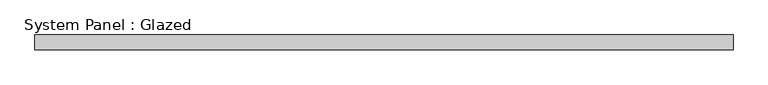
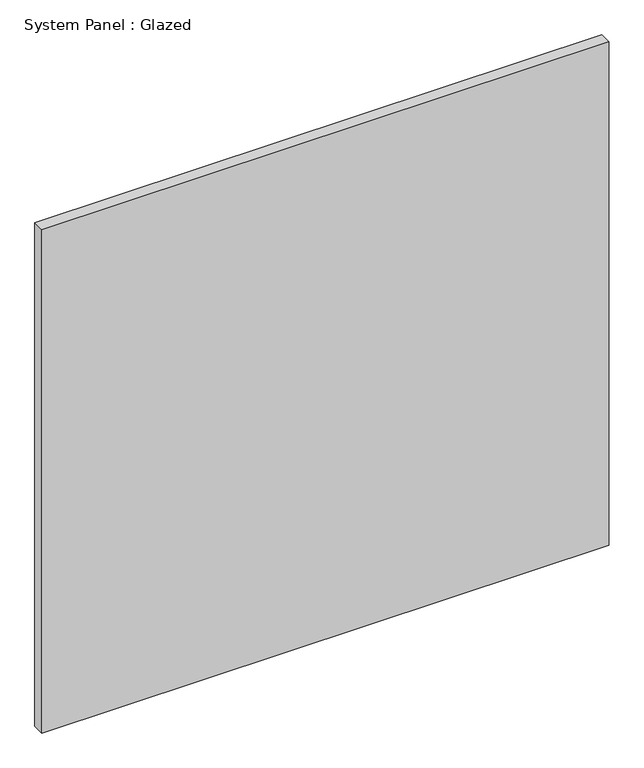
"""IFC4 building model written with IfcOpenShell, lengths in millimetres: plate geometry, System Panel : Glazed."""

from ifc_helpers import new_model, si_unit, origin, origin_with_axes, place, context, project, spatial, polyline, outline, extrude, source, transform, mapped, element, save


def system_panel_glazed_dc26df31(model_context):
    return source(origin(), model_context, "Body", "SweptSolid", [
        extrude(outline(polyline([(599.0166667, 19.05), (-599.0166667, 19.05), (-599.0166667, 44.45), (599.0166667, 44.45), (599.0166667, 19.05)])), origin_with_axes(), (0.0, 0.0, 1.0), 1123.95),
    ])


if __name__ == "__main__":
    model = new_model("IFC4")
    model_context = context("Model", 3, world=origin())
    ifc_project = project(units=[si_unit("LENGTHUNIT", "METRE", prefix="MILLI")], contexts=[model_context])
    site = spatial("IfcSite", under=ifc_project)
    building = spatial("IfcBuilding", under=site)
    placement = place(None, origin())
    system_panel_glazed_shape = system_panel_glazed_dc26df31(model_context)
    element("IfcPlate", 1, ObjectType="System Panel : Glazed", at=placement, inside=building, context=model_context, shape_type="MappedRepresentation", body=[
        mapped(system_panel_glazed_shape, transform((0.0, 0.0, 0.0), x_axis=(1.0, 0.0, 0.0), y_axis=(0.0, 1.0, 0.0), z_axis=(0.0, 0.0, 1.0))),
    ])
    save(model, "model.ifc")

# Revit data of these elements
# Element 1 (IfcPlate, "System Panel : Glazed")
#   Materials on its faces: "Glass"
# Materials
#   "Glass": class "Glass", colour RGB 218 227 224, transparency 0.85, Description = "Soda Lime Glass", Cost = 0
